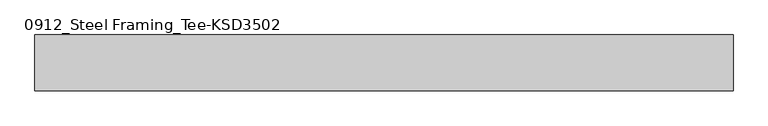
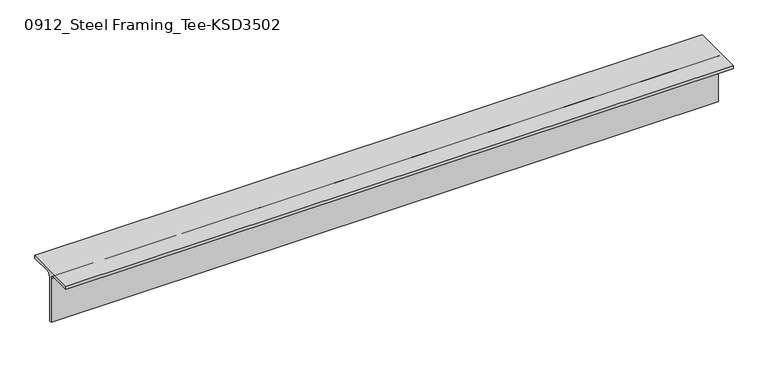
"""IFC4 building model written with IfcOpenShell, lengths in millimetres: member geometry, 0912_Steel Framing_Tee-KSD3502 : H_SB_ASB_CT-150x150x6.5x9."""

from ifc_helpers import new_model, si_unit, point, frame, frame_2d, origin, place, context, project, spatial, polyline, circle_curve, trimmed, segment, composite_curve, outline, extrude, source, transform, mapped, element, save


def member_0912_steel_framing_tee_ksd3502_ce33beac(model_context):
    return source(origin(), model_context, "Body", "SweptSolid", [
        extrude(outline(composite_curve([segment(polyline([(75.0, 75.0), (75.0, 66.0), (16.25, 66.0)]), True, "CONTINUOUS"), segment(trimmed(circle_curve(frame_2d((16.25, 53.0)), 13.0), [point((16.25, 66.0))], [point((3.25, 53.0))], True, "CARTESIAN"), True, "CONTINUOUS"), segment(polyline([(3.25, 53.0), (3.25, -75.0), (-3.25, -75.0), (-3.25, 53.0)]), True, "CONTINUOUS"), segment(trimmed(circle_curve(frame_2d((-16.25, 53.0)), 13.0), [point((-3.25, 53.0))], [point((-16.25, 66.0))], True, "CARTESIAN"), True, "CONTINUOUS"), segment(polyline([(-16.25, 66.0), (-75.0, 66.0), (-75.0, 75.0), (75.0, 75.0)]), True, "CONTINUOUS")], self_intersect=False)), frame((-1113.65, 0.0, 0.0), z_axis=(1.0, 0.0, 0.0), x_axis=(0.0, 1.0, 0.0)), (0.0, 0.0, 1.0), 1868.9),
    ])


if __name__ == "__main__":
    model = new_model("IFC4")
    model_context = context("Model", 3, world=origin())
    ifc_project = project(units=[si_unit("LENGTHUNIT", "METRE", prefix="MILLI")], contexts=[model_context])
    site = spatial("IfcSite", under=ifc_project)
    building = spatial("IfcBuilding", under=site)
    placement = place(None, origin())
    member_0912_steel_framing_tee_ksd3502_shape = member_0912_steel_framing_tee_ksd3502_ce33beac(model_context)
    element("IfcMember", 1, ObjectType="0912_Steel Framing_Tee-KSD3502 : H_SB_ASB_CT-150x150x6.5x9", at=placement, inside=building, context=model_context, shape_type="MappedRepresentation", body=[
        mapped(member_0912_steel_framing_tee_ksd3502_shape, transform((0.0, 0.0, 0.0), x_axis=(1.0, 0.0, 0.0), y_axis=(0.0, 1.0, 0.0), z_axis=(0.0, 0.0, 1.0))),
    ])
    save(model, "model.ifc")

# Revit data of these elements
# Type "0912_Steel Framing_Tee-KSD3502 : H_SB_ASB_CT-150x150x6.5x9"
#   H_WM Code_1 = "S01AA003-00001 | Main Steel Structure Fabrication Work | Shelter/Building | Light Steel - Standard (30KG/M>Weight) | Material: (   )"
#   H_WM Code_2 = "S03AA029-00001 | Main Steel Structure Erection Work | Shelter/Building | Light Steel (30KG/M>Weight) | Material: (   )"
#   H_WM Code_3 = "S01AA010-00001 | Main Steel Structure Fabrication Work | Shelter/Building | Steel Painting/Coating | for Non-Fireproofed Steel Surface, Surface Preparation, Primer, Second & Final Coat | Material: (   )"
#   H_Q'ty Cal Type Tag = "SB-Q2"
#   Width = 15.0 cm
#   Web Thickness = 0.65 cm
#   Web Fillet = 1.3 cm
#   Section Area = 23.39 cm²
#   Perimeter = 0.60 m²/m
#   Nominal Weight = 18.40 kgf/m
#   Height = 15.0 cm
#   Flange Thickness = 0.9 cm
#   Centroid Vertical = 7.5 cm
#   Centroid Horizontal = 7.5 cm
#   Length [instance default] = 1.5000 m
#   Structural Material [instance default] = Steel, 45-345
#   Warping Constant = (empty or 0)
#   Torsional Moment of Inertia = 0
#   Section Name Key = ""
#   Plastic Modulus weak axis = 0
#   Plastic Modulus strong axis = 0
#   Moment of Inertia weak axis = 0
#   Moment of Inertia strong axis = 0
#   Elastic Modulus weak axis = 0
#   Elastic Modulus strong axis = 0
#   Bolt Spacing = 0
#   Assembly Code = ""
# Element 1 (IfcMember, "0912_Steel Framing_Tee-KSD3502 : H_SB_ASB_CT-150x150x6.5x9")
#   Structural Material = none
# Materials
#   "Steel, 45-345": class "Metal", colour RGB 189 187 185, transparency 0, Description = "Steel 345 MPa", Cost = 0
